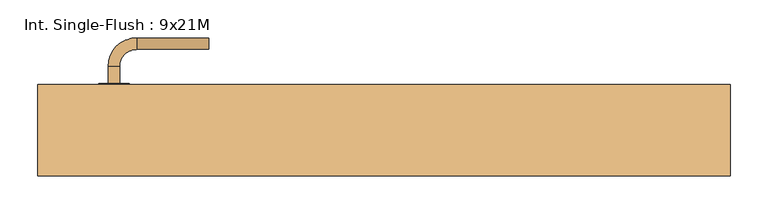
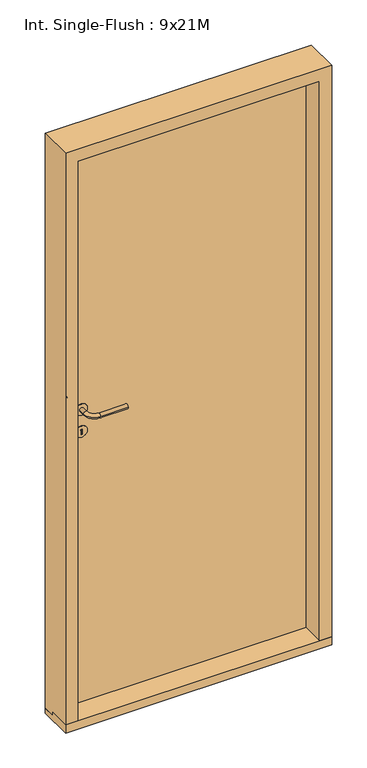
"""IFC4 building model written with IfcOpenShell, lengths in millimetres: door geometry, Int. Single-Flush : 9x21M."""

import ifcopenshell
import ifcopenshell.guid

model = None  # the IFC model being written
_history = None  # IfcOwnerHistory: only IFC2X3 demands one
_inside = {}  # id of a spatial element -> (the spatial element, [elements in it])
_under = {}  # id of a project, library or spatial element -> (it, [spatial elements below it])
_declared = {}  # id of a project -> (the project, [libraries it declares])
_typed = {}  # id of a type object -> (the type object, [elements of that type])
_made_of = {}  # id of a material, layer set ... -> (it, [elements and type objects made of it])


def new_model(schema):
    """Start an empty IFC model of exactly this schema.

    Asked for "IFC4X3", IfcOpenShell would pick the latest addendum, in which some entities
    have other attributes; the version numbers below select the first issue.
    IFC2X3 requires an IfcOwnerHistory on every rooted entity: one is made here for all.
    """
    global model, _history
    if schema == "IFC4X3":
        model = ifcopenshell.file(schema_version=(4, 3, 0, 0))
    else:
        model = ifcopenshell.file(schema=schema)
    _inside.clear()
    _under.clear()
    _declared.clear()
    _typed.clear()
    _made_of.clear()
    _history = None
    if model.schema == "IFC2X3":
        org = make("IfcOrganization", Name="unknown")
        user = make(
            "IfcPersonAndOrganization",
            ThePerson=make("IfcPerson", FamilyName="unknown"),
            TheOrganization=org,
        )
        app = make(
            "IfcApplication",
            ApplicationDeveloper=org,
            Version="unknown",
            ApplicationFullName="unknown",
            ApplicationIdentifier="unknown",
        )
        _history = make(
            "IfcOwnerHistory",
            OwningUser=user,
            OwningApplication=app,
            ChangeAction="ADDED",
            CreationDate=0,
        )
    return model


def make(cls, **values):
    """One entity of the class cls with the attributes given. An attribute that is None is left unset."""
    return model.create_entity(
        cls, **{name: value for name, value in values.items() if value is not None}
    )


def rooted(cls, **values):
    """An entity with a GlobalId (a new one), such as an element, a storey or a relation."""
    return make(cls, GlobalId=ifcopenshell.guid.new(), OwnerHistory=_history, **values)


def si_unit(unit_type, name, prefix=None):
    """IfcSIUnit, for example si_unit("LENGTHUNIT", "METRE", prefix="MILLI")."""
    return make("IfcSIUnit", UnitType=unit_type, Prefix=prefix, Name=name)


def assignment(units):
    """IfcUnitAssignment: the units of a project."""
    return None if units is None else make("IfcUnitAssignment", Units=units)


def point(xyz):
    """IfcCartesianPoint."""
    return None if xyz is None else make("IfcCartesianPoint", Coordinates=xyz)


def direction(xyz):
    """IfcDirection."""
    return None if xyz is None else make("IfcDirection", DirectionRatios=xyz)


def frame(location, z_axis=None, x_axis=None):
    """IfcAxis2Placement3D, a coordinate frame: its origin and axes. An axis left out is left unset."""
    return make(
        "IfcAxis2Placement3D",
        Location=point(location),
        Axis=direction(z_axis),
        RefDirection=direction(x_axis),
    )


def frame_2d(location, x_axis=None):
    """IfcAxis2Placement2D, a coordinate frame in the plane: its origin and x axis."""
    return make(
        "IfcAxis2Placement2D", Location=point(location), RefDirection=direction(x_axis)
    )


def origin():
    """The frame at (0, 0, 0) with its axes left unset."""
    return frame((0.0, 0.0, 0.0))


def place(relative_to, where):
    """IfcLocalPlacement: puts the frame where relative to a parent placement (None: the world)."""
    return make(
        "IfcLocalPlacement", PlacementRelTo=relative_to, RelativePlacement=where
    )


def context(
    kind, dimensions, precision=None, world=None, true_north=None, identifier=None
):
    """IfcGeometricRepresentationContext, for example the 3D "Model" context."""
    return make(
        "IfcGeometricRepresentationContext",
        ContextIdentifier=identifier,
        ContextType=kind,
        CoordinateSpaceDimension=dimensions,
        Precision=precision,
        WorldCoordinateSystem=world,
        TrueNorth=true_north,
    )


def project(units=None, contexts=None):
    """IfcProject with its units and contexts."""
    return rooted(
        "IfcProject",
        Name="project",
        RepresentationContexts=contexts,
        UnitsInContext=assignment(units),
    )


def spatial(cls, under=None, at=None, **own):
    """A site, building, storey or space (cls), placed at a placement, below another one or the project."""
    s = rooted(cls, ObjectPlacement=at, **own)
    if under is not None:
        _under.setdefault(under.id(), (under, []))[1].append(s)
    return s


def polyline(points):
    """IfcPolyline through the points."""
    return make("IfcPolyline", Points=[point(p) for p in points])


def circle_curve(where, radius):
    """IfcCircle in the frame where."""
    return make("IfcCircle", Position=where, Radius=radius)


def ellipse_curve(where, semi_axis1, semi_axis2):
    """IfcEllipse in the frame where."""
    return make(
        "IfcEllipse", Position=where, SemiAxis1=semi_axis1, SemiAxis2=semi_axis2
    )


def trimmed(basis, trim1, trim2, sense, master):
    """IfcTrimmedCurve: the piece of a basis curve between two trims."""
    return make(
        "IfcTrimmedCurve",
        BasisCurve=basis,
        Trim1=trim1,
        Trim2=trim2,
        SenseAgreement=sense,
        MasterRepresentation=master,
    )


def segment(curve, same_sense, transition):
    """IfcCompositeCurveSegment."""
    return make(
        "IfcCompositeCurveSegment",
        Transition=transition,
        SameSense=same_sense,
        ParentCurve=curve,
    )


def composite_curve(segments, self_intersect=None):
    """IfcCompositeCurve: segments joined end to end."""
    return make("IfcCompositeCurve", Segments=segments, SelfIntersect=self_intersect)


def outline(outer, holes=None, kind="AREA"):
    """IfcArbitraryClosedProfileDef: a profile drawn as a closed curve; with holes, ...WithVoids."""
    if holes is None:
        return make("IfcArbitraryClosedProfileDef", ProfileType=kind, OuterCurve=outer)
    return make(
        "IfcArbitraryProfileDefWithVoids",
        ProfileType=kind,
        OuterCurve=outer,
        InnerCurves=holes,
    )


def extrude(swept, where, along, depth):
    """IfcExtrudedAreaSolid: the profile swept, set in the frame where, extruded along a direction by depth."""
    return make(
        "IfcExtrudedAreaSolid",
        SweptArea=swept,
        Position=where,
        ExtrudedDirection=direction(along),
        Depth=depth,
    )


def faces_of(points, faces, orient=None, outer=None):
    """IfcFace entities. A face is a list of loops; a loop is a list of indices into points, from 0.

    orient and outer hold one flag for each loop. By default every Orientation is true, the
    first loop of a face is its IfcFaceOuterBound and the others are IfcFaceBound.
    """
    made = []
    for i, loops in enumerate(faces):
        bounds = []
        for j, loop in enumerate(loops):
            is_outer = j == 0 if outer is None else outer[i][j]
            bounds.append(
                make(
                    "IfcFaceOuterBound" if is_outer else "IfcFaceBound",
                    Bound=make("IfcPolyLoop", Polygon=[points[k] for k in loop]),
                    Orientation=True if orient is None else orient[i][j],
                )
            )
        made.append(make("IfcFace", Bounds=bounds))
    return made


def faceted_brep(points, faces, orient=None, outer=None, voids=None):
    """IfcFacetedBrep: a solid bounded by flat faces; with voids (closed shells), ...WithVoids."""
    shared = [point(p) for p in points]
    hull = make("IfcClosedShell", CfsFaces=faces_of(shared, faces, orient, outer))
    if voids is None:
        return make("IfcFacetedBrep", Outer=hull)
    return make(
        "IfcFacetedBrepWithVoids",
        Outer=hull,
        Voids=[
            make(cls, CfsFaces=faces_of(shared, fs, o, b)) for cls, fs, o, b in voids
        ],
    )


def shape(context_of_items, identifier, shape_type, items):
    """IfcShapeRepresentation: the items that make up one representation, for example the "Body"."""
    return make(
        "IfcShapeRepresentation",
        ContextOfItems=context_of_items,
        RepresentationIdentifier=identifier,
        RepresentationType=shape_type,
        Items=items,
    )


def source(mapping_origin, context_of_items, identifier, shape_type, items):
    """IfcRepresentationMap: a shape defined once, which mapped items show again and again."""
    return make(
        "IfcRepresentationMap",
        MappingOrigin=mapping_origin,
        MappedRepresentation=shape(context_of_items, identifier, shape_type, items),
    )


def transform(
    local_origin,
    x_axis=None,
    y_axis=None,
    z_axis=None,
    scale=None,
    scale2=None,
    scale3=None,
    uniform=True,
):
    """IfcCartesianTransformationOperator3D, or its non-uniform kind. x_axis, y_axis, z_axis: its Axis1, 2, 3."""
    if uniform:
        return make(
            "IfcCartesianTransformationOperator3D",
            Axis1=direction(x_axis),
            Axis2=direction(y_axis),
            LocalOrigin=point(local_origin),
            Scale=scale,
            Axis3=direction(z_axis),
        )
    return make(
        "IfcCartesianTransformationOperator3DnonUniform",
        Axis1=direction(x_axis),
        Axis2=direction(y_axis),
        LocalOrigin=point(local_origin),
        Scale=scale,
        Axis3=direction(z_axis),
        Scale2=scale2,
        Scale3=scale3,
    )


def mapped(mapping_source, mapping_target):
    """IfcMappedItem: shows the shape of a source again, moved by a transform."""
    return make(
        "IfcMappedItem", MappingSource=mapping_source, MappingTarget=mapping_target
    )


def made_of(thing, what):
    """Note that an element or type object is made of a material, layer set ...; save() writes the relation."""
    if what is not None:
        _made_of.setdefault(what.id(), (what, []))[1].append(thing)
    return thing


def element(
    cls,
    number,
    at=None,
    inside=None,
    cuts=None,
    type_object=None,
    material=None,
    context=None,
    identifier="Body",
    shape_type=None,
    held_by="IfcProductDefinitionShape",
    body=None,
    shapes=None,
    **own,
):
    """One element of the class cls, such as IfcWall. Its Tag is "e" and its number.

    at: its placement. inside: the storey or other place that contains it. cuts: it is an
    opening in that element (IfcRelVoidsElement). A single representation is given by context,
    identifier, shape_type and body (its items); several are given by shapes. held_by: the class
    of the entity that holds the representations. save() writes the other relations.
    """
    e = rooted(cls, Tag="e%d" % number, ObjectPlacement=at, **own)
    if body is not None:
        shapes = [shape(context, identifier, shape_type, body)]
    if shapes is not None:
        e.Representation = make(held_by, Representations=shapes)
    if inside is not None:
        _inside.setdefault(inside.id(), (inside, []))[1].append(e)
    if cuts is not None:
        rooted(
            "IfcRelVoidsElement", RelatingBuildingElement=cuts, RelatedOpeningElement=e
        )
    if type_object is not None:
        _typed.setdefault(type_object.id(), (type_object, []))[1].append(e)
    return made_of(e, material)


def aggregate(whole, parts):
    """IfcRelAggregates: a whole, such as a stair, and the parts it consists of."""
    return rooted("IfcRelAggregates", RelatingObject=whole, RelatedObjects=parts)


def save(model, path):
    """Write the relations noted so far, then the file.

    IfcRelAggregates (storeys below a building ...), IfcRelContainedInSpatialStructure (elements
    in a storey), IfcRelDefinesByType, IfcRelAssociatesMaterial and IfcRelDeclares: one each for
    every whole, place, type object, material and project.
    """
    for whole, parts in _under.values():
        aggregate(whole, parts)
    for where, things in _inside.values():
        rooted(
            "IfcRelContainedInSpatialStructure",
            RelatedElements=things,
            RelatingStructure=where,
        )
    for kind, things in _typed.values():
        rooted("IfcRelDefinesByType", RelatedObjects=things, RelatingType=kind)
    for what, things in _made_of.values():
        rooted("IfcRelAssociatesMaterial", RelatedObjects=things, RelatingMaterial=what)
    for by, libraries in _declared.values():
        rooted("IfcRelDeclares", RelatingContext=by, RelatedDefinitions=libraries)
    model.write(path)


def plane_surface(at):
    """IfcPlane: the flat surface through the origin of the frame at, square to its z axis."""
    return make("IfcPlane", Position=at)


def cylinder_surface(at, radius):
    """IfcCylindricalSurface: all points at the distance radius from the z axis of the frame at."""
    return make("IfcCylindricalSurface", Position=at, Radius=radius)


def revolved_surface(curve, axis_point, axis_direction):
    """IfcSurfaceOfRevolution: the curve turned about the line through axis_point along axis_direction."""
    return make(
        "IfcSurfaceOfRevolution",
        SweptCurve=make("IfcArbitraryOpenProfileDef", ProfileType="CURVE", Curve=curve),
        AxisPosition=make("IfcAxis1Placement", Location=point(axis_point), Axis=direction(axis_direction)),
    )


def advanced_brep(points, edges, surfaces, faces):
    """IfcAdvancedBrep: a solid bounded by faces that lie on surfaces and meet in shared edges.

    An edge is (start, end): straight between two places in points (the first is 0);
    or (start, end, curve); or (start, end, curve, False) where it runs against its curve.
    A face is (place in surfaces, loops), or (place, loops, False) where it looks against
    its surface's normal. A loop lists edges by number (the first is 1), with a minus sign
    where the edge is run from its end to its start. The first loop is the outer one.
    """
    corners = [point(p) for p in points]
    vertices = [make("IfcVertexPoint", VertexGeometry=c) for c in corners]
    made = []
    for start, end, *more in edges:
        made.append(
            make(
                "IfcEdgeCurve",
                EdgeStart=vertices[start],
                EdgeEnd=vertices[end],
                EdgeGeometry=more[0] if more else make("IfcPolyline", Points=[corners[start], corners[end]]),
                SameSense=more[1] if len(more) > 1 else True,
            )
        )
    hull = []
    for where, loops, *sense in faces:
        bounds = []
        for j, loop in enumerate(loops):
            ring = [make("IfcOrientedEdge", EdgeElement=made[abs(k) - 1], Orientation=k > 0) for k in loop]
            bounds.append(
                make(
                    "IfcFaceOuterBound" if j == 0 else "IfcFaceBound",
                    Bound=make("IfcEdgeLoop", EdgeList=ring),
                    Orientation=True,
                )
            )
        hull.append(make("IfcAdvancedFace", Bounds=bounds, FaceSurface=surfaces[where], SameSense=sense[0] if sense else True))
    return make("IfcAdvancedBrep", Outer=make("IfcClosedShell", CfsFaces=hull))


def int_single_flush_9x21m_be440b31(model_context):
    return source(origin(), model_context, "Body", "SolidModel", [
        extrude(outline(composite_curve([segment(trimmed(circle_curve(frame_2d((1090.0, -356.0)), 20.0), [point((1070.0, -356.0))], [point((1110.0, -356.0))], False, "CARTESIAN"), True, "CONTINUOUS"), segment(trimmed(circle_curve(frame_2d((1090.0, -356.0)), 20.0), [point((1110.0, -356.0))], [point((1070.0, -356.0))], False, "CARTESIAN"), True, "CONTINUOUS")], self_intersect=False)), frame((0.0, 60.0, 0.0), z_axis=(0.0, 1.0, 0.0), x_axis=(0.0, 0.0, 1.0)), (0.0, 0.0, 1.0), 2.0),
        advanced_brep(
        [(-363.5, 62.0, 1090.0), (-348.5, 62.0, 1090.0), (-363.5, 84.5, 1090.0), (-348.5, 84.5, 1090.0), (-326.0, 107.0, 1090.0), (-326.0, 122.0, 1090.0), (-231.0, 122.0, 1090.0), (-231.0, 107.0, 1090.0)],
        [
            (0, 1, circle_curve(frame((-356.0, 62.0, 1090.0), z_axis=(0.0, -1.0, 0.0), x_axis=(1.0, 0.0, 0.0)), 7.5)),
            (1, 0, circle_curve(frame((-356.0, 62.0, 1090.0), z_axis=(0.0, -1.0, 0.0), x_axis=(1.0, 0.0, 0.0)), 7.5)),
            (0, 2),
            (2, 3, circle_curve(frame((-356.0, 84.5, 1090.0), z_axis=(0.0, -1.0, 0.0), x_axis=(1.0, 0.0, 0.0)), 7.5)),
            (3, 1),
            (3, 2, circle_curve(frame((-356.0, 84.5, 1090.0), z_axis=(0.0, -1.0, 0.0), x_axis=(1.0, 0.0, 0.0)), 7.5)),
            (4, 3, circle_curve(frame((-326.0, 84.5, 1090.0), z_axis=(0.0, 0.0, 1.0), x_axis=(-1.0, 0.0, 0.0)), 22.5)),
            (2, 5, circle_curve(frame((-326.0, 84.5, 1090.0), z_axis=(0.0, 0.0, -1.0), x_axis=(-1.0, 0.0, 0.0)), 37.5)),
            (5, 4, circle_curve(frame((-326.0, 114.5, 1090.0), z_axis=(-1.0, 0.0, 0.0), x_axis=(0.0, -1.0, 0.0)), 7.5)),
            (4, 5, circle_curve(frame((-326.0, 114.5, 1090.0), z_axis=(-1.0, 0.0, 0.0), x_axis=(0.0, -1.0, 0.0)), 7.5)),
            (5, 6),
            (6, 7, circle_curve(frame((-231.0, 114.5, 1090.0), z_axis=(-1.0, 0.0, 0.0), x_axis=(0.0, -1.0, 0.0)), 7.5)),
            (7, 4),
            (7, 6, circle_curve(frame((-231.0, 114.5, 1090.0), z_axis=(-1.0, 0.0, 0.0), x_axis=(0.0, -1.0, 0.0)), 7.5)),
        ],
        [
            plane_surface(frame((-356.0, 62.0, 1090.0), z_axis=(0.0, -1.0, 0.0), x_axis=(0.0, 0.0, -1.0))),
            cylinder_surface(frame((-356.0, 62.0, 1090.0), z_axis=(0.0, -1.0, 0.0), x_axis=(1.0, 0.0, 0.0)), 7.5),
            revolved_surface(trimmed(ellipse_curve(frame((-356.0, 84.5, 1090.0), z_axis=(0.0, -1.0, 0.0), x_axis=(1.0, 0.0, 0.0)), 7.5, 7.5), [point((-363.5, 84.5, 1090.0))], [point((-348.5, 84.5, 1090.0))], True, "CARTESIAN"), (-326.0, 84.5, 1090.0), (0.0, 0.0, -1.0)),
            revolved_surface(trimmed(ellipse_curve(frame((-356.0, 84.5, 1090.0), z_axis=(0.0, -1.0, 0.0), x_axis=(1.0, 0.0, 0.0)), 7.5, 7.5), [point((-348.5, 84.5, 1090.0))], [point((-363.5, 84.5, 1090.0))], True, "CARTESIAN"), (-326.0, 84.5, 1090.0), (0.0, 0.0, -1.0)),
            cylinder_surface(frame((-326.0, 114.5, 1090.0), z_axis=(-1.0, 0.0, 0.0), x_axis=(0.0, -1.0, 0.0)), 7.5),
            plane_surface(frame((-231.0, 114.5, 1090.0), z_axis=(1.0, 0.0, 0.0), x_axis=(0.0, 0.0, -1.0))),
        ],
        [
            (0, [[1, 2]]),
            (1, [[-1, 3, 4, 5]]),
            (1, [[-2, -5, 6, -3]]),
            (2, [[7, -4, 8, 9]]),
            (3, [[-8, -6, -7, 10]]),
            (4, [[-9, 11, 12, 13]]),
            (4, [[-10, -13, 14, -11]]),
            (5, [[-14, -12]]),
        ],
    ),
        extrude(outline(composite_curve([segment(trimmed(circle_curve(frame_2d((1010.0, -356.0)), 20.0), [point((990.0, -356.0))], [point((1030.0, -356.0))], False, "CARTESIAN"), True, "CONTINUOUS"), segment(trimmed(circle_curve(frame_2d((1010.0, -356.0)), 20.0), [point((1030.0, -356.0))], [point((990.0, -356.0))], False, "CARTESIAN"), True, "CONTINUOUS")], self_intersect=False), holes=[composite_curve([segment(trimmed(circle_curve(frame_2d((1015.0, -356.0)), 3.0), [point((1012.4019238, -357.5))], [point((1012.4019238, -354.5))], True, "CARTESIAN"), True, "CONTINUOUS"), segment(polyline([(1012.4019238, -354.5), (1000.0, -354.5), (1000.0, -357.5), (1012.4019238, -357.5)]), True, "CONTINUOUS")], self_intersect=False)]), frame((0.0, 60.0, 0.0), z_axis=(0.0, 1.0, 0.0), x_axis=(0.0, 0.0, 1.0)), (0.0, 0.0, 1.0), 2.0),
        extrude(outline(composite_curve([segment(trimmed(circle_curve(frame_2d((1090.0, -356.0)), 20.0), [point((1070.0, -356.0))], [point((1110.0, -356.0))], False, "CARTESIAN"), True, "CONTINUOUS"), segment(trimmed(circle_curve(frame_2d((1090.0, -356.0)), 20.0), [point((1110.0, -356.0))], [point((1070.0, -356.0))], False, "CARTESIAN"), True, "CONTINUOUS")], self_intersect=False)), frame((0.0, 18.0, 0.0), z_axis=(0.0, 1.0, 0.0), x_axis=(0.0, 0.0, 1.0)), (0.0, 0.0, 1.0), 2.0),
        advanced_brep(
        [(-363.5, 18.0, 1090.0), (-348.5, 18.0, 1090.0), (-348.5, -4.5, 1090.0), (-363.5, -4.5, 1090.0), (-326.0, -27.0, 1090.0), (-326.0, -42.0, 1090.0), (-231.0, -27.0, 1090.0), (-231.0, -42.0, 1090.0)],
        [
            (0, 1, circle_curve(frame((-356.0, 18.0, 1090.0), z_axis=(0.0, 1.0, 0.0), x_axis=(1.0, 0.0, 0.0)), 7.5)),
            (1, 0, circle_curve(frame((-356.0, 18.0, 1090.0), z_axis=(0.0, 1.0, 0.0), x_axis=(1.0, 0.0, 0.0)), 7.5)),
            (1, 2),
            (2, 3, circle_curve(frame((-356.0, -4.5, 1090.0), z_axis=(0.0, 1.0, 0.0), x_axis=(1.0, 0.0, 0.0)), 7.5)),
            (3, 0),
            (3, 2, circle_curve(frame((-356.0, -4.5, 1090.0), z_axis=(0.0, 1.0, 0.0), x_axis=(1.0, 0.0, 0.0)), 7.5)),
            (4, 5, circle_curve(frame((-326.0, -34.5, 1090.0), z_axis=(-1.0, 0.0, 0.0), x_axis=(0.0, 1.0, 0.0)), 7.5)),
            (5, 3, circle_curve(frame((-326.0, -4.5, 1090.0), z_axis=(0.0, 0.0, -1.0), x_axis=(-1.0, 0.0, 0.0)), 37.5)),
            (2, 4, circle_curve(frame((-326.0, -4.5, 1090.0), z_axis=(0.0, 0.0, 1.0), x_axis=(-1.0, 0.0, 0.0)), 22.5)),
            (5, 4, circle_curve(frame((-326.0, -34.5, 1090.0), z_axis=(-1.0, 0.0, 0.0), x_axis=(0.0, 1.0, 0.0)), 7.5)),
            (4, 6),
            (6, 7, circle_curve(frame((-231.0, -34.5, 1090.0), z_axis=(-1.0, 0.0, 0.0), x_axis=(0.0, 1.0, 0.0)), 7.5)),
            (7, 5),
            (7, 6, circle_curve(frame((-231.0, -34.5, 1090.0), z_axis=(-1.0, 0.0, 0.0), x_axis=(0.0, 1.0, 0.0)), 7.5)),
        ],
        [
            plane_surface(frame((-356.0, 18.0, 1090.0), z_axis=(0.0, 1.0, 0.0), x_axis=(0.0, 0.0, -1.0))),
            cylinder_surface(frame((-356.0, 18.0, 1090.0), z_axis=(0.0, 1.0, 0.0), x_axis=(1.0, 0.0, 0.0)), 7.5),
            revolved_surface(trimmed(ellipse_curve(frame((-356.0, -4.5, 1090.0), z_axis=(0.0, -1.0, 0.0), x_axis=(1.0, 0.0, 0.0)), 7.5, 7.5), [point((-363.5, -4.5, 1090.0))], [point((-348.5, -4.5, 1090.0))], True, "CARTESIAN"), (-326.0, -4.5, 1090.0), (0.0, 0.0, -1.0)),
            revolved_surface(trimmed(ellipse_curve(frame((-356.0, -4.5, 1090.0), z_axis=(0.0, -1.0, 0.0), x_axis=(1.0, 0.0, 0.0)), 7.5, 7.5), [point((-348.5, -4.5, 1090.0))], [point((-363.5, -4.5, 1090.0))], True, "CARTESIAN"), (-326.0, -4.5, 1090.0), (0.0, 0.0, -1.0)),
            cylinder_surface(frame((-326.0, -34.5, 1090.0), z_axis=(-1.0, 0.0, 0.0), x_axis=(0.0, 1.0, 0.0)), 7.5),
            plane_surface(frame((-231.0, -34.5, 1090.0), z_axis=(1.0, 0.0, 0.0), x_axis=(0.0, 0.0, -1.0))),
        ],
        [
            (0, [[1, 2]]),
            (1, [[3, 4, 5, -2]]),
            (1, [[-5, 6, -3, -1]]),
            (2, [[7, 8, -4, 9]]),
            (3, [[10, -9, -6, -8]]),
            (4, [[11, 12, 13, -7]]),
            (4, [[-13, 14, -11, -10]]),
            (5, [[-12, -14]]),
        ],
    ),
        extrude(outline(composite_curve([segment(trimmed(circle_curve(frame_2d((1010.0, -356.0)), 20.0), [point((990.0, -356.0))], [point((1030.0, -356.0))], False, "CARTESIAN"), True, "CONTINUOUS"), segment(trimmed(circle_curve(frame_2d((1010.0, -356.0)), 20.0), [point((1030.0, -356.0))], [point((990.0, -356.0))], False, "CARTESIAN"), True, "CONTINUOUS")], self_intersect=False), holes=[composite_curve([segment(trimmed(circle_curve(frame_2d((1015.0, -356.0)), 3.0), [point((1012.4019238, -357.5))], [point((1012.4019238, -354.5))], True, "CARTESIAN"), True, "CONTINUOUS"), segment(polyline([(1012.4019238, -354.5), (1000.0, -354.5), (1000.0, -357.5), (1012.4019238, -357.5)]), True, "CONTINUOUS")], self_intersect=False)]), frame((0.0, 18.0, 0.0), z_axis=(0.0, 1.0, 0.0), x_axis=(0.0, 0.0, 1.0)), (0.0, 0.0, 1.0), 2.0),
        extrude(outline(polyline([(426.0, 20.0), (-426.0, 20.0), (-426.0, 60.0), (426.0, 60.0), (426.0, 20.0)])), frame((0.0, 0.0, 18.0), z_axis=(0.0, 0.0, 1.0), x_axis=(1.0, 0.0, 0.0)), (0.0, 0.0, 1.0), 2052.0),
        faceted_brep([(-426.0, 20.0, 2070.0), (426.0, 20.0, 2070.0), (426.0, 20.0, 30.0), (414.0, 20.0, 30.0), (414.0, 20.0, 2058.0), (-414.0, 20.0, 2058.0), (-414.0, 20.0, 30.0), (-426.0, 20.0, 30.0), (-426.0, 60.0, 2070.0), (-426.0, 20.0, 18.0), (-426.0, 60.0, 18.0), (-456.0, 20.0, 30.0), (-456.0, 20.0, 18.0), (456.0, 20.0, 30.0), (426.0, 20.0, 18.0), (456.0, 20.0, 18.0), (-456.0, 60.0, 18.0), (426.0, 60.0, 18.0), (456.0, 60.0, 18.0), (-456.0, 60.0, 2100.0), (456.0, 60.0, 2100.0), (426.0, 60.0, 2070.0), (-414.0, -60.0, 30.0), (-456.0, -60.0, 30.0), (456.0, -60.0, 30.0), (414.0, -60.0, 30.0), (414.0, -60.0, 2058.0), (-414.0, -60.0, 2058.0), (456.0, -60.0, 2100.0), (-456.0, -60.0, 2100.0)], [[[0, 1, 2, 3, 4, 5, 6, 7]], [[8, 0, 7, 9, 10]], [[7, 11, 12, 9]], [[13, 2, 14, 15]], [[9, 12, 16, 10]], [[15, 14, 17, 18]], [[19, 20, 18, 17, 21, 8, 10, 16]], [[1, 21, 17, 14, 2]], [[11, 7, 6, 22, 23]], [[2, 13, 24, 25, 3]], [[26, 4, 3, 25]], [[5, 27, 22, 6]], [[27, 26, 25, 24, 28, 29, 23, 22]], [[20, 28, 24, 13, 15, 18]], [[29, 19, 16, 12, 11, 23]], [[0, 8, 21, 1]], [[5, 4, 26, 27]], [[29, 28, 20, 19]]]),
        extrude(outline(polyline([(20.0, 30.0), (20.0, 18.0), (60.0, 18.0), (60.0, 0.0), (-60.0, 0.0), (-60.0, 30.0), (20.0, 30.0)])), frame((-456.0, 0.0, 0.0), z_axis=(1.0, 0.0, 0.0), x_axis=(0.0, 1.0, 0.0)), (0.0, 0.0, 1.0), 912.0),
    ])


if __name__ == "__main__":
    model = new_model("IFC4")
    model_context = context("Model", 3, world=origin())
    ifc_project = project(units=[si_unit("LENGTHUNIT", "METRE", prefix="MILLI")], contexts=[model_context])
    site = spatial("IfcSite", under=ifc_project)
    building = spatial("IfcBuilding", under=site)
    placement = place(None, origin())
    int_single_flush_9x21m_shape = int_single_flush_9x21m_be440b31(model_context)
    element("IfcDoor", 1, ObjectType="Int. Single-Flush : 9x21M", at=placement, inside=building, context=model_context, shape_type="MappedRepresentation", body=[
        mapped(int_single_flush_9x21m_shape, transform((0.0, 0.0, 0.0), x_axis=(1.0, 0.0, 0.0), y_axis=(0.0, 1.0, 0.0), z_axis=(0.0, 0.0, 1.0))),
    ])
    save(model, "model.ifc")

# Revit data of these elements
# Type "Int. Single-Flush : 9x21M"
#   Type Mark = "53"
#   Sound Rating = ""
#   Hinge Side [instance default] = ""
#   Creator Build [instance default] = "2017.0301.0"
#   Creator Organization [instance default] = "© Danish Educational Content"
#   Creator Name [instance default] = "© Erik Falck Jørgensen"
#   Analytic Construction = "<None>"
#   length#3 = 18 mm
#   length#2 = 42 mm
#   length#1 = 0 mm
#   length#4 = 912 mm
#   Thickness = 40 mm
#   Seal Width = 12 mm
#   Rough Width = 912 mm
#   Rough Height = 2100 mm
#   Rabbet Width = 12 mm
#   Rabbet Depth = 40 mm
#   Interior Distance [instance default] = 0 mm
#   Height = 2088 mm
#   Width = 888 mm
#   Handle From Side = 100 mm
#   Handle From Bottom = 1090 mm
#   Exterior Direction [instance default] = 0.00°
#   Case Depth [instance default] = 200 mm
#   Case Width = 30 mm
#   Exterior Distance [instance default] = 0 mm
#   Threshold = yes
#   Sealing = no
#   Hinging = yes
#   Wall Closure = 1
#   Door Panel = no
#   Panel = none
#   Handle Finish = none
#   Handle = element 510752
#   Case/Transom = none
#   Function = (empty or 0)
#   Assembly Code = ""
# Element 1 (IfcDoor, "Int. Single-Flush : 9x21M")
#   Case Depth = 120 mm
#   Materials on its faces: "Stainless Steel, Polished", "Default Frame/Mullion (Interior/Exterior)", "Default Door Panel (Exterior/Interior)"
# Materials
#   "Stainless Steel, Polished": class "Metal", colour RGB 180 180 180, transparency 0, Description = "Rustfri stål, poleret", Cost = 0
#   "Default Frame/Mullion (Interior/Exterior)": class "Generic", colour RGB 205 205 205, transparency 0, Description = "Udefineret karm/ramme materiale", Cost = 0
#   "Default Door Panel (Exterior/Interior)": class "Generic", colour RGB 205 205 205, transparency 0, Description = "Udefineret dørplade materiale", Cost = 0
